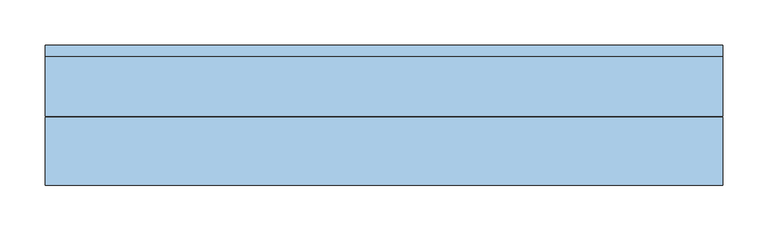
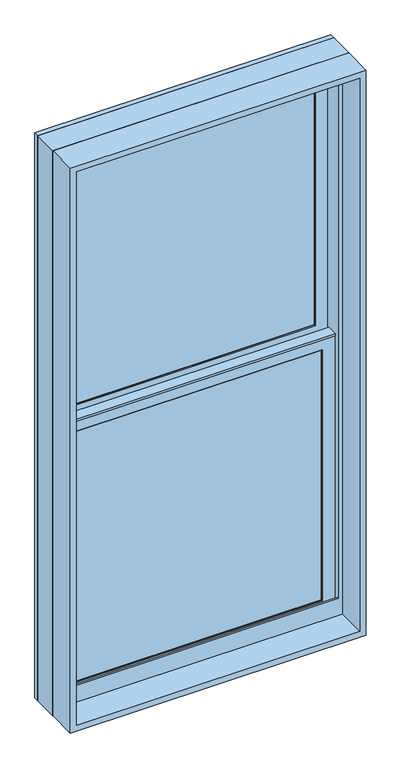
"""IFC4 building model written with IfcOpenShell, lengths in millimetres: window geometry, Window-Double_Hung-Marvin-Essential : ESDH2650."""

from ifc_helpers import new_model, si_unit, frame, origin, place, context, project, spatial, polyline, outline, extrude, faceted_brep, source, transform, mapped, element, save


def window_1745e17a(model_context):
    return source(origin(), model_context, "Body", "SolidModel", [
        extrude(outline(polyline([(115.3583333, 20.6375), (115.3583333, 15.875), (96.3083333, 15.875), (96.3083333, 20.6375), (115.3583333, 20.6375)])), frame((0.0, 0.0, 984.25), z_axis=(0.0, 0.0, 1.0), x_axis=(1.0, 0.0, 0.0)), (0.0, 0.0, 1.0), 679.45),
        extrude(outline(polyline([(-96.3083333, 20.6375), (-96.3083333, 15.875), (-115.3583333, 15.875), (-115.3583333, 20.6375), (-96.3083333, 20.6375)])), frame((0.0, 0.0, 984.25), z_axis=(0.0, 0.0, 1.0), x_axis=(1.0, 0.0, 0.0)), (0.0, 0.0, 1.0), 679.45),
        extrude(outline(polyline([(317.5, 20.6375), (317.5, 15.875), (-317.5, 15.875), (-317.5, 20.6375), (317.5, 20.6375)])), frame((0.0, 0.0, 1314.45), z_axis=(0.0, 0.0, 1.0), x_axis=(1.0, 0.0, 0.0)), (0.0, 0.0, 1.0), 19.05),
        extrude(outline(polyline([(-115.3583333, 46.83125), (-115.3583333, 51.59375), (-96.3083333, 51.59375), (-96.3083333, 46.83125), (-115.3583333, 46.83125)])), frame((0.0, 0.0, 1701.8), z_axis=(0.0, 0.0, 1.0), x_axis=(1.0, 0.0, 0.0)), (0.0, 0.0, 1.0), 679.45),
        extrude(outline(polyline([(96.3083333, 46.83125), (96.3083333, 51.59375), (115.3583333, 51.59375), (115.3583333, 46.83125), (96.3083333, 46.83125)])), frame((0.0, 0.0, 1701.8), z_axis=(0.0, 0.0, 1.0), x_axis=(1.0, 0.0, 0.0)), (0.0, 0.0, 1.0), 679.45),
        extrude(outline(polyline([(-317.5, 46.83125), (-317.5, 51.59375), (317.5, 51.59375), (317.5, 46.83125), (-317.5, 46.83125)])), frame((0.0, 0.0, 2032.0), z_axis=(0.0, 0.0, 1.0), x_axis=(1.0, 0.0, 0.0)), (0.0, 0.0, 1.0), 19.05),
        extrude(outline(polyline([(115.3583333, 20.6375), (96.3083333, 20.6375), (96.3083333, 25.4), (115.3583333, 25.4), (115.3583333, 20.6375)])), frame((0.0, 0.0, 984.25), z_axis=(0.0, 0.0, 1.0), x_axis=(1.0, 0.0, 0.0)), (0.0, 0.0, 1.0), 679.45),
        extrude(outline(polyline([(-96.3083333, 20.6375), (-115.3583333, 20.6375), (-115.3583333, 25.4), (-96.3083333, 25.4), (-96.3083333, 20.6375)])), frame((0.0, 0.0, 984.25), z_axis=(0.0, 0.0, 1.0), x_axis=(1.0, 0.0, 0.0)), (0.0, 0.0, 1.0), 679.45),
        extrude(outline(polyline([(317.5, 20.6375), (-317.5, 20.6375), (-317.5, 25.4), (317.5, 25.4), (317.5, 20.6375)])), frame((0.0, 0.0, 1314.45), z_axis=(0.0, 0.0, 1.0), x_axis=(1.0, 0.0, 0.0)), (0.0, 0.0, 1.0), 19.05),
        extrude(outline(polyline([(-115.3583333, 56.35625), (-96.3083333, 56.35625), (-96.3083333, 51.59375), (-115.3583333, 51.59375), (-115.3583333, 56.35625)])), frame((0.0, 0.0, 1701.8), z_axis=(0.0, 0.0, 1.0), x_axis=(1.0, 0.0, 0.0)), (0.0, 0.0, 1.0), 679.45),
        extrude(outline(polyline([(96.3083333, 56.35625), (115.3583333, 56.35625), (115.3583333, 51.59375), (96.3083333, 51.59375), (96.3083333, 56.35625)])), frame((0.0, 0.0, 1701.8), z_axis=(0.0, 0.0, 1.0), x_axis=(1.0, 0.0, 0.0)), (0.0, 0.0, 1.0), 679.45),
        extrude(outline(polyline([(-317.5, 56.35625), (317.5, 56.35625), (317.5, 51.59375), (-317.5, 51.59375), (-317.5, 56.35625)])), frame((0.0, 0.0, 2032.0), z_axis=(0.0, 0.0, 1.0), x_axis=(1.0, 0.0, 0.0)), (0.0, 0.0, 1.0), 19.05),
        faceted_brep([(-344.4875, 5.6780605, 1693.7351748), (-344.4875, 5.6780605, 1689.1), (344.4875, 5.6780605, 1689.1), (344.4875, 5.6780605, 1693.7351748), (-344.4875, 34.8118605, 1693.7351748), (344.4875, 34.8118605, 1693.7351748), (344.4875, 34.8118605, 1689.1), (-344.4875, 34.8118605, 1689.1), (-344.4875, 30.1625, 1689.1), (-344.4875, 30.1625, 957.2625), (-344.4875, 8.9241104, 957.2625), (-344.4875, 8.9241104, 1689.1), (344.4875, 8.9241104, 1689.1), (344.4875, 30.1625, 1689.1), (344.4875, 8.9241104, 957.2625), (344.4875, 30.1625, 957.2625), (-328.6034752, 11.90625, 1674.8034752), (-328.6034752, 30.1625, 1674.8034752), (328.6034752, 30.1625, 1674.8034752), (328.6034752, 11.90625, 1674.8034752), (-311.94375, 10.4662439, 1658.14375), (-311.94375, 11.90625, 1658.14375), (311.94375, 11.90625, 1658.14375), (311.94375, 10.4662439, 1658.14375), (313.4858834, 8.9241104, 1659.6858834), (-313.4858834, 8.9241104, 1659.6858834), (328.6034752, 30.1625, 973.1465248), (328.6034752, 11.90625, 973.1465248), (311.94375, 11.90625, 989.80625), (311.94375, 10.4662439, 989.80625), (313.4858834, 8.9241104, 988.2641166), (-328.6034752, 30.1625, 973.1465248), (-328.6034752, 11.90625, 973.1465248), (-311.94375, 11.90625, 989.80625), (-311.94375, 10.4662439, 989.80625), (-313.4858834, 8.9241104, 988.2641166)], [[[0, 1, 2, 3]], [[4, 5, 6, 7]], [[1, 0, 4, 7, 8, 9, 10, 11]], [[2, 1, 11, 12]], [[7, 6, 13, 8]], [[3, 2, 12, 14, 15, 13, 6, 5]], [[0, 3, 5, 4]], [[16, 17, 18, 19]], [[20, 21, 22, 23]], [[20, 23, 24, 25]], [[19, 18, 26, 27]], [[23, 22, 28, 29]], [[24, 23, 29, 30]], [[27, 26, 31, 32]], [[29, 28, 33, 34]], [[30, 29, 34, 35]], [[15, 14, 10, 9]], [[15, 9, 8, 13], [18, 17, 31, 26]], [[17, 16, 32, 31]], [[16, 19, 27, 32], [22, 21, 33, 28]], [[21, 20, 34, 33]], [[20, 25, 35, 34]], [[10, 14, 12, 11], [25, 24, 30, 35]]]),
        extrude(outline(polyline([(38.5955581, 1674.8125), (33.5778968, 1674.8125), (33.5778968, 1676.4), (39.9405976, 1676.4), (39.9405976, 1674.8125), (61.515625, 1674.8125), (47.6307501, 1671.4975159), (38.5955581, 1671.4975159), (38.5955581, 1674.8125)])), frame((-344.4875, 0.0, 0.0), z_axis=(1.0, 0.0, 0.0), x_axis=(0.0, 1.0, 0.0)), (0.0, 0.0, 1.0), 688.975),
        faceted_brep([(374.65, 0.0, 927.1), (374.65, 0.0, 2438.4), (-374.65, 0.0, 2438.4), (-374.65, 0.0, 927.1), (348.45625, 0.0, 988.21875), (-348.45625, 0.0, 988.21875), (-348.45625, 0.0, 2412.20625), (348.45625, 0.0, 2412.20625), (348.45625, 3.96875, 927.1), (-348.45625, 3.96875, 927.1), (-348.45625, 3.96875, 988.21875), (348.45625, 3.96875, 988.21875), (-374.65, 65.6828125, 927.1), (-348.45625, 65.6828125, 927.1), (348.45625, 65.6828125, 927.1), (374.65, 65.6828125, 927.1), (-374.65, 65.6828125, 2438.4), (374.65, 65.6828125, 2438.4), (348.45625, 65.6828125, 2412.20625), (-348.45625, 65.6828125, 2412.20625)], [[[0, 1, 2, 3], [4, 5, 6, 7]], [[8, 9, 10, 11]], [[5, 4, 11, 10]], [[0, 3, 12, 13, 9, 8, 14, 15]], [[13, 12, 16, 17, 15, 14, 18, 19]], [[13, 19, 6, 5, 10, 9]], [[7, 6, 19, 18]], [[18, 14, 8, 11, 4, 7]], [[1, 0, 15, 17]], [[2, 1, 17, 16]], [[3, 2, 16, 12]]]),
        faceted_brep([(348.45625, 30.1625, 1682.75), (346.86875, 30.1625, 1682.75), (346.86875, 30.1625, 951.4544613), (348.45625, 30.1625, 951.4544613), (-346.86875, 30.1625, 1682.75), (-348.45625, 30.1625, 1682.75), (-348.45625, 30.1625, 951.4544613), (-346.86875, 30.1625, 951.4544613), (346.86875, 63.5, 1682.75), (348.45625, 63.5, 1682.75), (348.45625, 63.5, 944.9743077), (346.86875, 63.5, 944.9743077), (-348.45625, 63.5, 1682.75), (-346.86875, 63.5, 1682.75), (-346.86875, 63.5, 944.9743077), (-348.45625, 63.5, 944.9743077), (359.7108932, 3.96875, 956.5460105), (359.7108932, 3.96875, 927.1), (359.7108932, 65.6828125, 927.1), (359.7108932, 65.6828125, 944.550012), (-359.7108932, 3.96875, 927.1), (-359.7108932, 3.96875, 956.5460105), (-359.7108932, 65.6828125, 944.550012), (-359.7108932, 65.6828125, 927.1), (359.7108932, 78.58125, 942.0428097), (-359.7108932, 78.58125, 942.0428097), (-357.6971252, 68.2348864, 944.0539391), (-339.73135, 68.2348864, 944.0539391), (-339.73135, 65.6828125, 944.550012), (339.73135, 65.6828125, 944.550012), (339.73135, 68.2348864, 944.0539391), (357.6971252, 68.2348864, 944.0539391), (-374.65, 65.6828125, 927.1), (-374.65, 78.5948249, 927.1), (374.65, 78.5948249, 927.1), (374.65, 65.6828125, 927.1), (-374.65, 78.58125, 2438.4), (374.65, 78.58125, 2438.4), (359.7108932, 78.58125, 2423.4608932), (-359.7108932, 78.58125, 2423.4608932), (-374.65, 65.6828125, 2438.4), (-357.6971252, 68.2348864, 2421.4471252), (357.6971252, 68.2348864, 2421.4471252), (339.73135, 68.2348864, 2403.48135), (-339.73135, 68.2348864, 2403.48135), (-339.73135, 65.6828125, 2403.48135), (339.73135, 65.6828125, 2403.48135), (374.65, 65.6828125, 2438.4)], [[[0, 1, 2, 3]], [[4, 5, 6, 7]], [[8, 9, 10, 11]], [[12, 13, 14, 15]], [[1, 8, 11, 2]], [[9, 0, 3, 10]], [[1, 0, 9, 8]], [[5, 4, 13, 12]], [[5, 12, 15, 6]], [[13, 4, 7, 14]], [[16, 17, 18, 19]], [[20, 21, 22, 23]], [[24, 25, 26, 27, 28, 22, 21, 16, 19, 29, 30, 31], [3, 2, 11, 10], [7, 6, 15, 14]], [[17, 16, 21, 20]], [[17, 20, 23, 32, 33, 34, 35, 18]], [[34, 33, 36, 37], [25, 24, 38, 39]], [[33, 32, 40, 36]], [[39, 41, 26, 25]], [[41, 42, 31, 30, 43, 44, 27, 26]], [[44, 45, 28, 27]], [[40, 32, 23, 22, 28, 45, 46, 29, 19, 18, 35, 47]], [[36, 40, 47, 37]], [[39, 38, 42, 41]], [[44, 43, 46, 45]], [[34, 37, 47, 35]], [[42, 38, 24, 31]], [[46, 43, 30, 29]]]),
        extrude(outline(polyline([(324.64375, 11.90625), (-324.64375, 11.90625), (-324.64375, 15.08125), (324.64375, 15.08125), (324.64375, 11.90625)])), frame((0.0, 0.0, 977.10625), z_axis=(0.0, 0.0, 1.0), x_axis=(1.0, 0.0, 0.0)), (0.0, 0.0, 1.0), 693.7375),
        extrude(outline(polyline([(324.64375, 42.8625), (-324.64375, 42.8625), (-324.64375, 46.0375), (324.64375, 46.0375), (324.64375, 42.8625)])), frame((0.0, 0.0, 1694.65625), z_axis=(0.0, 0.0, 1.0), x_axis=(1.0, 0.0, 0.0)), (0.0, 0.0, 1.0), 693.7375),
        faceted_brep([(-311.94375, 31.194477, 1658.14375), (-313.4858834, 32.7366104, 1659.6858834), (313.4858834, 32.7366104, 1659.6858834), (311.94375, 31.194477, 1658.14375), (-311.94375, 30.1625, 1658.14375), (311.94375, 30.1625, 1658.14375), (-344.4875, 32.7366104, 1690.6875), (-344.4875, 30.1625, 1690.6875), (344.4875, 30.1625, 1690.6875), (344.4875, 32.7366104, 1690.6875), (313.4858834, 32.7366104, 988.2641166), (311.94375, 31.194477, 989.80625), (311.94375, 30.1625, 989.80625), (344.4875, 30.1625, 957.2625), (344.4875, 32.7366104, 957.2625), (-313.4858834, 32.7366104, 988.2641166), (-311.94375, 31.194477, 989.80625), (-311.94375, 30.1625, 989.80625), (-344.4875, 30.1625, 957.2625), (-344.4875, 32.7366104, 957.2625)], [[[0, 1, 2, 3]], [[4, 0, 3, 5]], [[6, 7, 8, 9]], [[3, 2, 10, 11]], [[5, 3, 11, 12]], [[9, 8, 13, 14]], [[11, 10, 15, 16]], [[12, 11, 16, 17]], [[14, 13, 18, 19]], [[9, 14, 19, 6], [1, 15, 10, 2]], [[16, 15, 1, 0]], [[17, 16, 0, 4]], [[7, 18, 13, 8], [5, 12, 17, 4]], [[19, 18, 7, 6]]]),
        faceted_brep([(-328.6034752, 42.8625, 2392.3534752), (-328.6034752, 61.11875, 2392.3534752), (328.6034752, 61.11875, 2392.3534752), (328.6034752, 42.8625, 2392.3534752), (-311.94375, 41.4224939, 2375.69375), (-311.94375, 42.8625, 2375.69375), (311.94375, 42.8625, 2375.69375), (311.94375, 41.4224939, 2375.69375), (-313.4858834, 39.8803604, 2377.2358834), (313.4858834, 39.8803604, 2377.2358834), (-344.4875, 61.11875, 2408.2375), (-344.4875, 39.8803604, 2408.2375), (344.4875, 39.8803604, 2408.2375), (344.4875, 61.11875, 2408.2375), (328.6034752, 61.11875, 1690.6965248), (328.6034752, 42.8625, 1690.6965248), (311.94375, 42.8625, 1707.35625), (311.94375, 41.4224939, 1707.35625), (313.4858834, 39.8803604, 1705.8141166), (344.4875, 39.8803604, 1674.8125), (344.4875, 61.11875, 1674.8125), (-328.6034752, 61.11875, 1690.6965248), (-328.6034752, 42.8625, 1690.6965248), (-311.94375, 42.8625, 1707.35625), (-311.94375, 41.4224939, 1707.35625), (-313.4858834, 39.8803604, 1705.8141166), (-344.4875, 39.8803604, 1674.8125), (-344.4875, 61.11875, 1674.8125)], [[[0, 1, 2, 3]], [[4, 5, 6, 7]], [[8, 4, 7, 9]], [[10, 11, 12, 13]], [[3, 2, 14, 15]], [[7, 6, 16, 17]], [[9, 7, 17, 18]], [[13, 12, 19, 20]], [[15, 14, 21, 22]], [[17, 16, 23, 24]], [[18, 17, 24, 25]], [[20, 19, 26, 27]], [[13, 20, 27, 10], [1, 21, 14, 2]], [[22, 21, 1, 0]], [[3, 15, 22, 0], [5, 23, 16, 6]], [[24, 23, 5, 4]], [[25, 24, 4, 8]], [[11, 26, 19, 12], [9, 18, 25, 8]], [[27, 26, 11, 10]]]),
        faceted_brep([(-344.4875, 61.11875, 1674.8125), (-344.4875, 63.6928604, 1674.8125), (344.4875, 63.6928604, 1674.8125), (344.4875, 61.11875, 1674.8125), (-311.94375, 62.150727, 1707.35625), (-311.94375, 61.11875, 1707.35625), (311.94375, 61.11875, 1707.35625), (311.94375, 62.150727, 1707.35625), (-313.4858834, 63.6928604, 1705.8141166), (313.4858834, 63.6928604, 1705.8141166), (344.4875, 63.6928604, 2408.2375), (344.4875, 61.11875, 2408.2375), (311.94375, 61.11875, 2375.69375), (311.94375, 62.150727, 2375.69375), (313.4858834, 63.6928604, 2377.2358834), (-344.4875, 63.6928604, 2408.2375), (-344.4875, 61.11875, 2408.2375), (-311.94375, 61.11875, 2375.69375), (-311.94375, 62.150727, 2375.69375), (-313.4858834, 63.6928604, 2377.2358834)], [[[0, 1, 2, 3]], [[4, 5, 6, 7]], [[8, 4, 7, 9]], [[3, 2, 10, 11]], [[7, 6, 12, 13]], [[9, 7, 13, 14]], [[11, 10, 15, 16]], [[13, 12, 17, 18]], [[14, 13, 18, 19]], [[16, 15, 1, 0]], [[3, 11, 16, 0], [5, 17, 12, 6]], [[18, 17, 5, 4]], [[19, 18, 4, 8]], [[1, 15, 10, 2], [9, 14, 19, 8]]]),
        extrude(outline(polyline([(324.64375, 26.19375), (-324.64375, 26.19375), (-324.64375, 30.1625), (324.64375, 30.1625), (324.64375, 26.19375)])), frame((0.0, 0.0, 977.10625), z_axis=(0.0, 0.0, 1.0), x_axis=(1.0, 0.0, 0.0)), (0.0, 0.0, 1.0), 693.7375),
        extrude(outline(polyline([(324.64375, 57.15), (-324.64375, 57.15), (-324.64375, 61.11875), (324.64375, 61.11875), (324.64375, 57.15)])), frame((0.0, 0.0, 1694.65625), z_axis=(0.0, 0.0, 1.0), x_axis=(1.0, 0.0, 0.0)), (0.0, 0.0, 1.0), 693.7375),
        extrude(outline(polyline([(2438.4, 374.65), (2438.4, -374.65), (927.1, -374.65), (927.1, 374.65), (2438.4, 374.65)]), holes=[polyline([(2422.525, 358.775), (942.975, 358.775), (942.975, -358.775), (2422.525, -358.775), (2422.525, 358.775)])]), frame((0.0, -76.2, 0.0), z_axis=(0.0, 1.0, 0.0), x_axis=(0.0, 0.0, 1.0)), (0.0, 0.0, 1.0), 75.40625),
    ])


if __name__ == "__main__":
    model = new_model("IFC4")
    model_context = context("Model", 3, world=origin())
    ifc_project = project(units=[si_unit("LENGTHUNIT", "METRE", prefix="MILLI")], contexts=[model_context])
    site = spatial("IfcSite", under=ifc_project)
    building = spatial("IfcBuilding", under=site)
    placement = place(None, origin())
    window_shape = window_1745e17a(model_context)
    element("IfcWindow", 1, ObjectType="Window-Double_Hung-Marvin-Essential : ESDH2650", at=placement, inside=building, context=model_context, shape_type="MappedRepresentation", body=[
        mapped(window_shape, transform((0.0, 0.0, 0.0), x_axis=(1.0, 0.0, 0.0), y_axis=(0.0, 1.0, 0.0), z_axis=(0.0, 0.0, 1.0))),
    ])
    save(model, "model.ifc")

# Revit data of these elements
# Type "Window-Double_Hung-Marvin-Essential : ESDH2650"
#   Type Mark = "63"
#   Window Type = "Essential Double Hung"
#   Product data url = "https://bimobject.com/marvin-windows-and-doors/product/marvin-dhwau"
#   Product Guid = "c4a96547-874c-4385-91dc-a058adc19d98"
#   Frame = "All Ultrex"
#   Egress Window = "No"
#   URL = "www.marvin.com"
#   Model = "ESDH2650"
#   Manufacturer = "Marvin Windows and Doors"
#   Label Egress = ""
#   Glass Type = "IG Low E II with Argon"
#   Design Pressure = "DP50"
#   Description = "3060 DBHG"
#   Analytic Construction = "<None>"
#   Prairie Corner Width = 0' - 4"
#   Prairie Corner Height = 0' - 4"
#   Egress Width = 2' - 2 9/16"
#   Egress Height = 2' - 1 27/128"
#   Rough Width = 2' - 6"
#   Rough Height = 5' - 0"
#   Nominal Width = 2' - 6"
#   Nominal Height = 5' - 0"
#   Inset to Installation Flange [instance default] = 0' - 1"
#   Height = 4' - 11 1/2"
#   Egress Area = 4.65046 SF
#   Default Head Height = 8' - 0"
#   Width = 2' - 5 1/2"
#   Daylight Area = 8.9764 SF
#   DLO Width = 2' - 0 9/16"
#   DLO Height = 2' - 2 5/16"
#   Muntins Top Sash = yes
#   Lites Wide Top Sash = 3
#   Lites Wide Bottom Sash = 3
#   Lites High Top Sash = 2
#   Lites High Bottom Sash = 2
#   Lite Cut Prairie 9 = no
#   Lite Cut HV Grid = yes
#   Muntins Bottom Sash = yes
#   Label Visibility = no
#   Jamb Extension Visibility = yes
#   Edition number = 1
#   Interior Material = Ultrex-Marvin-Stonewhite
#   Glazing Material = Glass-Marvin-IG Low E II with Argon
#   Cladding Material = Ultrex-Marvin-Pebblegray
#   Wall Closure = (empty or 0)
#   Assembly Code = ""
# Element 1 (IfcWindow, "Window-Double_Hung-Marvin-Essential : ESDH2650")
#   Materials on its faces: "Ultrex-Marvin-Pebblegray", "Ultrex-Marvin-Stonewhite", "Glass-Marvin-IG Low E II with Argon"
# Materials
#   "Ultrex-Marvin-Stonewhite": class "Paint", colour RGB 250 251 245, transparency 0
#   "Glass-Marvin-IG Low E II with Argon": class "Glass", colour RGB 0 128 192, transparency 0.85
#   "Ultrex-Marvin-Pebblegray": class "Paint", colour RGB 189 185 173, transparency 0
